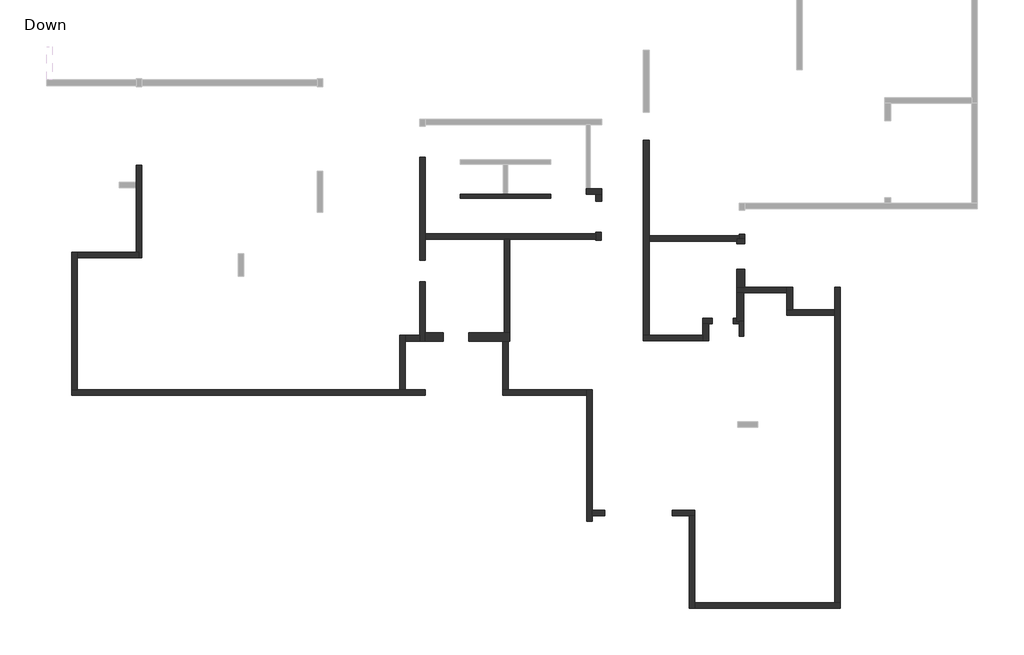
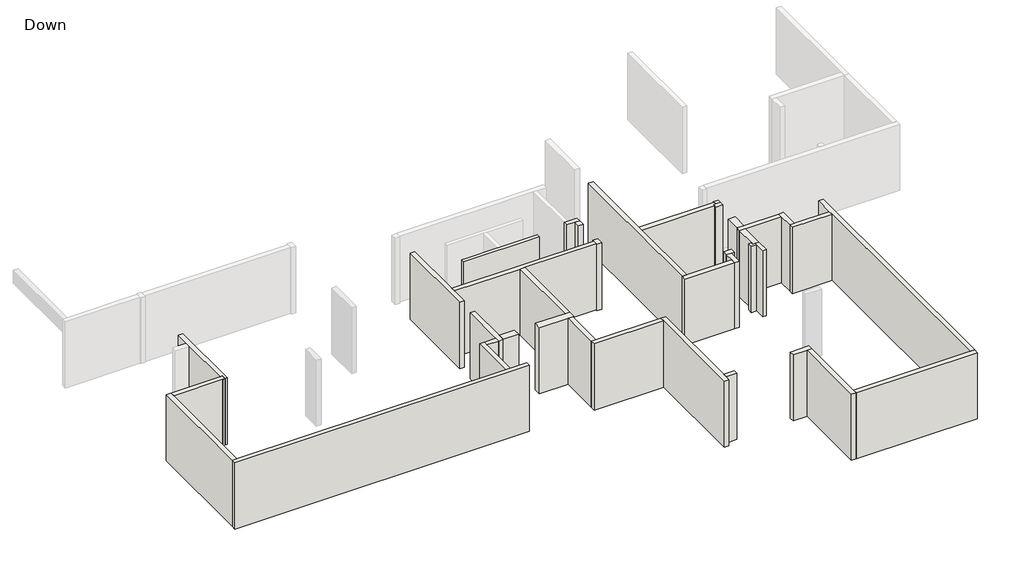
# One storey, part 1 of 3: 38 walls.
"""IFC4 building model written with IfcOpenShell, lengths in millimetres."""

from ifc_helpers import new_model, si_unit, origin, place, context, project, spatial, faceted_brep, element, save

model = new_model("IFC4")

# Units and contexts
model_context = context("Model", 3, world=origin())
ifc_project = project(units=[si_unit("LENGTHUNIT", "METRE", prefix="MILLI")], contexts=[model_context])

# Site, building, storey
site = spatial("IfcSite", under=ifc_project)
building = spatial("IfcBuilding", under=site)
storey = spatial("IfcBuildingStorey", under=building, Name="Down", Elevation=0.0)

# Walls
placement = place(None, origin())
element("IfcWall", 1, ObjectType="15", at=placement, inside=storey, context=model_context, shape_type="Brep", body=[
    faceted_brep([(8929.8987326, -5377.2065162, 0.0), (8929.8987326, -4829.2179242, 0.0), (8929.8987326, -4829.2179242, 3000.0), (8929.8987326, -5377.2065162, 3000.0), (8929.8987326, -5377.2065162, 2800.0), (8779.8987326, -5377.2065162, 0.0), (8779.8987326, -5377.2065162, 2800.0), (8779.8987326, -5377.2065162, 3000.0), (8779.8987326, -4929.2179242, 3000.0), (8779.8987326, -4829.2179242, 3000.0), (8779.8987326, -4829.2179242, 0.0), (8779.8987326, -4929.2179242, 0.0)], [[[0, 1, 2, 3, 4]], [[5, 6, 7, 8, 9, 10, 11]], [[1, 0, 5, 11, 10]], [[2, 1, 10, 9]], [[3, 2, 9, 8, 7]], [[0, 4, 3, 7, 6, 5]]]),
])
element("IfcWall", 2, ObjectType="15", at=placement, inside=storey, context=model_context, shape_type="Brep", body=[
    faceted_brep([(2055.2627374, -306.6458737, 0.0), (511.0080091, -306.6458737, 0.0), (361.0080091, -306.6458737, 0.0), (-1185.5058006, -306.6458737, 0.0), (-1185.5058006, -306.6458737, 2800.0), (-1185.5058006, -306.6458737, 3000.0), (-985.5058006, -306.6458737, 3000.0), (361.0080091, -306.6458737, 3000.0), (511.0080091, -306.6458737, 3000.0), (1795.2627374, -306.6458737, 3000.0), (2055.2627374, -306.6458737, 3000.0), (2055.2627374, -306.6458737, 2800.0), (2055.2627374, -456.6458737, 0.0), (2055.2627374, -456.6458737, 2800.0), (2055.2627374, -456.6458737, 3000.0), (-1185.5058006, -456.6458737, 3000.0), (-1185.5058006, -456.6458737, 2800.0), (-1185.5058006, -456.6458737, 0.0)], [[[0, 1, 2, 3, 4, 5, 6, 7, 8, 9, 10, 11]], [[12, 13, 14, 15, 16, 17]], [[3, 2, 1, 0, 12, 17]], [[5, 4, 3, 17, 16, 15]], [[10, 9, 8, 7, 6, 5, 15, 14]], [[0, 11, 10, 14, 13, 12]]]),
])
element("IfcWall", 3, ObjectType="20", at=placement, inside=storey, context=model_context, shape_type="Brep", body=[
    faceted_brep([(3525.3580541, -11777.7243787, 0.0), (3983.0434339, -11777.7243787, 0.0), (3983.0434339, -11777.7243787, 2800.0), (3983.0434339, -11777.7243787, 3000.0), (3525.3580541, -11777.7243787, 3000.0), (3525.3580541, -11777.7243787, 2800.0), (3525.3580541, -11577.7243787, 0.0), (3525.3580541, -11577.7243787, 2800.0), (3525.3580541, -11577.7243787, 3000.0), (3983.0434339, -11577.7243787, 3000.0), (3983.0434339, -11577.7243787, 2800.0), (3983.0434339, -11577.7243787, 0.0)], [[[0, 1, 2, 3, 4, 5]], [[6, 7, 8, 9, 10, 11]], [[1, 0, 6, 11]], [[3, 2, 1, 11, 10, 9]], [[4, 3, 9, 8]], [[0, 5, 4, 8, 7, 6]]]),
])
element("IfcWall", 4, ObjectType="20", at=placement, inside=storey, context=model_context, shape_type="Brep", body=[
    faceted_brep([(6385.0248209, -11777.7243787, 0.0), (6985.0248209, -11777.7243787, 0.0), (7185.0248209, -11777.7243787, 0.0), (7185.0248209, -11777.7243787, 3000.0), (6985.0248209, -11777.7243787, 3000.0), (6385.0248209, -11777.7243787, 3000.0), (6385.0248209, -11777.7243787, 2800.0), (6385.0248209, -11577.7243787, 0.0), (6385.0248209, -11577.7243787, 2800.0), (6385.0248209, -11577.7243787, 3000.0), (7185.0248209, -11577.7243787, 3000.0), (7185.0248209, -11577.7243787, 2800.0), (7185.0248209, -11577.7243787, 0.0)], [[[0, 1, 2, 3, 4, 5, 6]], [[7, 8, 9, 10, 11, 12]], [[2, 1, 0, 7, 12]], [[5, 4, 3, 10, 9]], [[0, 6, 5, 9, 8, 7]], [[3, 2, 12, 11, 10]]]),
])
element("IfcWall", 5, ObjectType="20", at=placement, inside=storey, context=model_context, shape_type="Brep", body=[
    faceted_brep([(6985.0248209, -11777.7243787, 0.0), (6985.0248209, -15077.7243787, 0.0), (6985.0248209, -15077.7243787, 3000.0), (6985.0248209, -14877.7243787, 3000.0), (6985.0248209, -11777.7243787, 3000.0), (6985.0248209, -11777.7243787, 2800.0), (7185.0248209, -11777.7243787, 0.0), (7185.0248209, -11777.7243787, 3000.0), (7185.0248209, -14877.7243787, 3000.0), (7185.0248209, -15077.7243787, 3000.0), (7185.0248209, -15077.7243787, 0.0), (7185.0248209, -14877.7243787, 0.0)], [[[0, 1, 2, 3, 4, 5]], [[6, 7, 8, 9, 10, 11]], [[1, 0, 6, 11, 10]], [[4, 3, 2, 9, 8, 7]], [[0, 5, 4, 7, 6]], [[2, 1, 10, 9]]]),
])
element("IfcWall", 6, ObjectType="20", at=placement, inside=storey, context=model_context, shape_type="Brep", body=[
    faceted_brep([(7185.0248209, -15077.7243787, 0.0), (12385.0248209, -15077.7243787, 0.0), (12385.0248209, -15077.7243787, 3000.0), (7185.0248209, -15077.7243787, 3000.0), (7185.0248209, -14877.7243787, 0.0), (7185.0248209, -14877.7243787, 2800.0), (7185.0248209, -14877.7243787, 3000.0), (12185.0248209, -14877.7243787, 3000.0), (12385.0248209, -14877.7243787, 3000.0), (12385.0248209, -14877.7243787, 0.0), (12185.0248209, -14877.7243787, 0.0)], [[[0, 1, 2, 3]], [[4, 5, 6, 7, 8, 9, 10]], [[1, 0, 4, 10, 9]], [[3, 2, 8, 7, 6]], [[0, 3, 6, 5, 4]], [[2, 1, 9, 8]]]),
])
element("IfcWall", 7, ObjectType="20", at=placement, inside=storey, context=model_context, shape_type="Brep", body=[
    faceted_brep([(12385.0248209, -14877.7243787, 0.0), (12385.0248209, -3627.7243787, 0.0), (12385.0248209, -3627.7243787, 3000.0), (12385.0248209, -14877.7243787, 3000.0), (12185.0248209, -14877.7243787, 0.0), (12185.0248209, -14877.7243787, 2800.0), (12185.0248209, -14877.7243787, 3000.0), (12185.0248209, -4626.5873327, 3000.0), (12185.0248209, -4426.5873327, 3000.0), (12185.0248209, -3627.7243787, 3000.0), (12185.0248209, -3627.7243787, 0.0), (12185.0248209, -4426.5873327, 0.0), (12185.0248209, -4626.5873327, 0.0)], [[[0, 1, 2, 3]], [[4, 5, 6, 7, 8, 9, 10, 11, 12]], [[1, 0, 4, 12, 11, 10]], [[2, 1, 10, 9]], [[3, 2, 9, 8, 7, 6]], [[0, 3, 6, 5, 4]]]),
])
element("IfcWall", 8, ObjectType="20", at=placement, inside=storey, context=model_context, shape_type="Brep", body=[
    faceted_brep([(10478.8780181, -4626.5873327, 0.0), (12185.0248209, -4626.5873327, 0.0), (12185.0248209, -4626.5873327, 2800.0), (12185.0248209, -4626.5873327, 3000.0), (10478.8780181, -4626.5873327, 3000.0), (10478.8780181, -4626.5873327, 2800.0), (10478.8780181, -4426.5873327, 0.0), (10478.8780181, -4426.5873327, 3000.0), (10678.8780181, -4426.5873327, 3000.0), (12185.0248209, -4426.5873327, 3000.0), (12185.0248209, -4426.5873327, 0.0), (10678.8780181, -4426.5873327, 0.0)], [[[0, 1, 2, 3, 4, 5]], [[6, 7, 8, 9, 10, 11]], [[1, 0, 6, 11, 10]], [[4, 3, 9, 8, 7]], [[3, 2, 1, 10, 9]], [[0, 5, 4, 7, 6]]]),
])
element("IfcWall", 9, ObjectType="20", at=placement, inside=storey, context=model_context, shape_type="Brep", body=[
    faceted_brep([(10678.8780181, -4426.5873327, 0.0), (10678.8780181, -3625.7617548, 0.0), (10678.8780181, -3625.7617548, 3000.0), (10678.8780181, -4426.5873327, 3000.0), (10478.8780181, -4426.5873327, 0.0), (10478.8780181, -4426.5873327, 3000.0), (10478.8780181, -3825.7617548, 3000.0), (10478.8780181, -3625.7617548, 3000.0), (10478.8780181, -3625.7617548, 0.0), (10478.8780181, -3825.7617548, 0.0)], [[[0, 1, 2, 3]], [[4, 5, 6, 7, 8, 9]], [[1, 0, 4, 9, 8]], [[3, 2, 7, 6, 5]], [[2, 1, 8, 7]], [[0, 3, 5, 4]]]),
])
element("IfcWall", 10, ObjectType="20", at=placement, inside=storey, context=model_context, shape_type="Brep", body=[
    faceted_brep([(10478.8780181, -3625.7617548, 0.0), (8979.7748959, -3625.7617548, 0.0), (8679.9812904, -3625.7617548, 0.0), (8679.9812904, -3625.7617548, 2800.0), (8679.9812904, -3625.7617548, 3000.0), (8979.7748959, -3625.7617548, 3000.0), (10478.8780181, -3625.7617548, 3000.0), (10478.8780181, -3825.7617548, 0.0), (10478.8780181, -3825.7617548, 2800.0), (10478.8780181, -3825.7617548, 3000.0), (8929.9812904, -3825.7617548, 3000.0), (8679.9812904, -3825.7617548, 3000.0), (8679.9812904, -3825.7617548, 0.0), (8929.9812904, -3825.7617548, 0.0)], [[[0, 1, 2, 3, 4, 5, 6]], [[7, 8, 9, 10, 11, 12, 13]], [[2, 1, 0, 7, 13, 12]], [[6, 5, 4, 11, 10, 9]], [[0, 6, 9, 8, 7]], [[4, 3, 2, 12, 11]]]),
])
element("IfcWall", 11, ObjectType="20", at=placement, inside=storey, context=model_context, shape_type="Brep", body=[
    faceted_brep([(8679.9812904, -4729.2179242, 0.0), (8554.8987326, -4729.2179242, 0.0), (8554.8987326, -4729.2179242, 2800.0), (8554.8987326, -4729.2179242, 3000.0), (8679.9812904, -4729.2179242, 3000.0), (8779.8987326, -4929.2179242, 0.0), (8779.8987326, -4929.2179242, 2800.0), (8779.8987326, -4929.2179242, 3000.0), (8554.8987326, -4929.2179242, 3000.0), (8554.8987326, -4929.2179242, 2800.0), (8554.8987326, -4929.2179242, 0.0), (8679.9812904, -4829.2179242, 0.0), (8779.8987326, -4829.2179242, 0.0), (8779.8987326, -4829.2179242, 3000.0), (8679.9812904, -4829.2179242, 3000.0)], [[[0, 1, 2, 3, 4]], [[5, 6, 7, 8, 9, 10]], [[1, 0, 11, 12, 5, 10]], [[3, 2, 1, 10, 9, 8]], [[4, 3, 8, 7, 13, 14]], [[0, 4, 14, 11]], [[14, 13, 12, 11]], [[13, 7, 6, 5, 12]]]),
])
element("IfcWall", 12, ObjectType="20", at=placement, inside=storey, context=model_context, shape_type="Brep", body=[
    faceted_brep([(7481.1671205, -4929.2179242, 0.0), (7481.1671205, -5329.7132709, 0.0), (7481.1671205, -5529.7132709, 0.0), (7481.1671205, -5529.7132709, 3000.0), (7481.1671205, -5329.7132709, 3000.0), (7481.1671205, -4929.2179242, 3000.0), (7681.1671205, -4929.2179242, 0.0), (7681.1671205, -4929.2179242, 2800.0), (7681.1671205, -4929.2179242, 3000.0), (7681.1671205, -5529.7132709, 3000.0), (7681.1671205, -5529.7132709, 2800.0), (7681.1671205, -5529.7132709, 0.0)], [[[0, 1, 2, 3, 4, 5]], [[6, 7, 8, 9, 10, 11]], [[2, 1, 0, 6, 11]], [[5, 4, 3, 9, 8]], [[3, 2, 11, 10, 9]], [[0, 5, 8, 7, 6]]]),
])
element("IfcWall", 13, ObjectType="20", at=placement, inside=storey, context=model_context, shape_type="Brep", body=[
    faceted_brep([(7481.1671205, -5329.7132709, 0.0), (5555.6042265, -5329.7132709, 0.0), (5355.6042265, -5329.7132709, 0.0), (5355.6042265, -5329.7132709, 3000.0), (5555.6042265, -5329.7132709, 3000.0), (7481.1671205, -5329.7132709, 3000.0), (7481.1671205, -5329.7132709, 2800.0), (7481.1671205, -5529.7132709, 0.0), (7481.1671205, -5529.7132709, 3000.0), (5355.6042265, -5529.7132709, 3000.0), (5355.6042265, -5529.7132709, 2800.0), (5355.6042265, -5529.7132709, 0.0)], [[[0, 1, 2, 3, 4, 5, 6]], [[7, 8, 9, 10, 11]], [[2, 1, 0, 7, 11]], [[5, 4, 3, 9, 8]], [[0, 6, 5, 8, 7]], [[3, 2, 11, 10, 9]]]),
])
element("IfcWall", 14, ObjectType="20", at=placement, inside=storey, context=model_context, shape_type="Brep", body=[
    faceted_brep([(5555.6042265, -5329.7132709, 0.0), (5555.6042265, -1979.0002718, 0.0), (5555.6042265, -1779.0002718, 0.0), (5555.6042265, 1623.6415775, 0.0), (5555.6042265, 1623.6415775, 2800.0), (5555.6042265, 1623.6415775, 3000.0), (5555.6042265, -1779.0002718, 3000.0), (5555.6042265, -1979.0002718, 3000.0), (5555.6042265, -5329.7132709, 3000.0), (5555.6042265, -5329.7132709, 2800.0), (5355.6042265, -5329.7132709, 0.0), (5355.6042265, -5329.7132709, 3000.0), (5355.6042265, -1955.5013225, 3000.0), (5355.6042265, -560.9043547, 3000.0), (5355.6042265, 1623.6415775, 3000.0), (5355.6042265, 1623.6415775, 2800.0), (5355.6042265, 1623.6415775, 0.0)], [[[0, 1, 2, 3, 4, 5, 6, 7, 8, 9]], [[10, 11, 12, 13, 14, 15, 16]], [[3, 2, 1, 0, 10, 16]], [[5, 4, 3, 16, 15, 14]], [[8, 7, 6, 5, 14, 13, 12, 11]], [[0, 9, 8, 11, 10]]]),
])
element("IfcWall", 15, ObjectType="20", at=placement, inside=storey, context=model_context, shape_type="Brep", body=[
    faceted_brep([(5555.6042265, -1979.0002718, 0.0), (8679.7748959, -1979.0002718, 0.0), (8679.7748959, -1979.0002718, 2800.0), (8679.7748959, -1979.0002718, 3000.0), (5555.6042265, -1979.0002718, 3000.0), (5555.6042265, -1979.0002718, 2800.0), (5555.6042265, -1779.0002718, 0.0), (5555.6042265, -1779.0002718, 2800.0), (5555.6042265, -1779.0002718, 3000.0), (8779.7748959, -1779.0002718, 3000.0), (8779.7748959, -1779.0002718, 2800.0), (8779.7748959, -1779.0002718, 0.0), (8779.7748959, -1879.0002718, 0.0), (8679.7748959, -1879.0002718, 0.0), (8679.7748959, -1879.0002718, 3000.0), (8779.7748959, -1879.0002718, 3000.0)], [[[0, 1, 2, 3, 4, 5]], [[6, 7, 8, 9, 10, 11]], [[1, 0, 6, 11, 12, 13]], [[4, 3, 14, 15, 9, 8]], [[3, 2, 1, 13, 14]], [[13, 12, 15, 14]], [[12, 11, 10, 9, 15]], [[0, 5, 4, 8, 7, 6]]]),
])
element("IfcWall", 16, ObjectType="20", at=placement, inside=storey, context=model_context, shape_type="Brep", body=[
    faceted_brep([(3525.3580541, -11977.8894943, 0.0), (3525.3580541, -11777.7243787, 0.0), (3525.3580541, -11577.7243787, 0.0), (3525.3580541, -7276.5573117, 0.0), (3525.3580541, -7276.5573117, 2800.0), (3525.3580541, -7276.5573117, 3000.0), (3525.3580541, -11577.7243787, 3000.0), (3525.3580541, -11777.7243787, 3000.0), (3525.3580541, -11977.8894943, 3000.0), (3525.3580541, -11977.8894943, 2400.0), (3325.3580541, -11977.8894943, 0.0), (3325.3580541, -11977.8894943, 2400.0), (3325.3580541, -11977.8894943, 3000.0), (3325.3580541, -7476.5573117, 3000.0), (3325.3580541, -7276.5573117, 3000.0), (3325.3580541, -7276.5573117, 0.0), (3325.3580541, -7476.5573117, 0.0)], [[[0, 1, 2, 3, 4, 5, 6, 7, 8, 9]], [[10, 11, 12, 13, 14, 15, 16]], [[3, 2, 1, 0, 10, 16, 15]], [[8, 7, 6, 5, 14, 13, 12]], [[0, 9, 8, 12, 11, 10]], [[5, 4, 3, 15, 14]]]),
])
element("IfcWall", 17, ObjectType="20", at=placement, inside=storey, context=model_context, shape_type="Brep", body=[
    faceted_brep([(3325.3580541, -7276.5573117, 0.0), (539.5617467, -7276.5573117, 0.0), (339.5617467, -7276.5573117, 0.0), (339.5617467, -7276.5573117, 3000.0), (539.5617467, -7276.5573117, 3000.0), (3325.3580541, -7276.5573117, 3000.0), (3325.3580541, -7476.5573117, 0.0), (3325.3580541, -7476.5573117, 3000.0), (339.5617467, -7476.5573117, 3000.0), (339.5617467, -7476.5573117, 0.0)], [[[0, 1, 2, 3, 4, 5]], [[6, 7, 8, 9]], [[2, 1, 0, 6, 9]], [[5, 4, 3, 8, 7]], [[3, 2, 9, 8]], [[0, 5, 7, 6]]]),
])
element("IfcWall", 18, ObjectType="20", at=placement, inside=storey, context=model_context, shape_type="Brep", body=[
    faceted_brep([(539.5617467, -7276.5573117, 0.0), (539.5617467, -5546.2285816, 0.0), (539.5617467, -5546.2285816, 2800.0), (539.5617467, -5546.2285816, 3000.0), (539.5617467, -7276.5573117, 3000.0), (539.5617467, -7276.5573117, 2800.0), (339.5617467, -7276.5573117, 0.0), (339.5617467, -7276.5573117, 3000.0), (339.5617467, -5546.2285816, 3000.0), (339.5617467, -5546.2285816, 0.0)], [[[0, 1, 2, 3, 4, 5]], [[6, 7, 8, 9]], [[1, 0, 6, 9]], [[4, 3, 8, 7]], [[0, 5, 4, 7, 6]], [[3, 2, 1, 9, 8]]]),
])
element("IfcWall", 19, ObjectType="20", at=placement, inside=storey, context=model_context, shape_type="Brep", body=[
    faceted_brep([(-2431.7719369, -7276.5573117, 0.0), (-3134.897875, -7276.5573117, 0.0), (-3334.897875, -7276.5573117, 0.0), (-14851.7058906, -7276.5573117, 0.0), (-15051.7058906, -7276.5573117, 0.0), (-15051.7058906, -7276.5573117, 3000.0), (-14851.7058906, -7276.5573117, 3000.0), (-3334.897875, -7276.5573117, 3000.0), (-3134.897875, -7276.5573117, 3000.0), (-2431.7719369, -7276.5573117, 3000.0), (-2431.7719369, -7476.5573117, 0.0), (-2431.7719369, -7476.5573117, 3000.0), (-15051.7058906, -7476.5573117, 3000.0), (-15051.7058906, -7476.5573117, 0.0)], [[[0, 1, 2, 3, 4, 5, 6, 7, 8, 9]], [[10, 11, 12, 13]], [[4, 3, 2, 1, 0, 10, 13]], [[9, 8, 7, 6, 5, 12, 11]], [[0, 9, 11, 10]], [[5, 4, 13, 12]]]),
])
element("IfcWall", 20, ObjectType="20", at=placement, inside=storey, context=model_context, shape_type="Brep", body=[
    faceted_brep([(-14851.7058906, -7276.5573117, 0.0), (-14851.7058906, -2576.5573117, 0.0), (-14851.7058906, -2376.5573117, 0.0), (-14851.7058906, -2376.5573117, 3000.0), (-14851.7058906, -2576.5573117, 3000.0), (-14851.7058906, -7276.5573117, 3000.0), (-14851.7058906, -7276.5573117, 2800.0), (-15051.7058906, -7276.5573117, 0.0), (-15051.7058906, -7276.5573117, 3000.0), (-15051.7058906, -2376.5573117, 3000.0), (-15051.7058906, -2376.5573117, 0.0)], [[[0, 1, 2, 3, 4, 5, 6]], [[7, 8, 9, 10]], [[2, 1, 0, 7, 10]], [[5, 4, 3, 9, 8]], [[0, 6, 5, 8, 7]], [[3, 2, 10, 9]]]),
])
element("IfcWall", 21, ObjectType="20", at=placement, inside=storey, context=model_context, shape_type="Brep", body=[
    faceted_brep([(-14851.7058906, -2576.5573117, 0.0), (-12744.8761098, -2576.5573117, 0.0), (-12645.0412254, -2576.5573117, 0.0), (-12645.0412254, -2576.5573117, 3000.0), (-12744.8761098, -2576.5573117, 3000.0), (-14851.7058906, -2576.5573117, 3000.0), (-14851.7058906, -2576.5573117, 2800.0), (-14851.7058906, -2376.5573117, 0.0), (-14851.7058906, -2376.5573117, 3000.0), (-12744.8761098, -2376.5573117, 3000.0), (-12645.0412254, -2376.5573117, 3000.0), (-12645.0412254, -2376.5573117, 0.0), (-12744.8761098, -2376.5573117, 0.0)], [[[0, 1, 2, 3, 4, 5, 6]], [[7, 8, 9, 10, 11, 12]], [[2, 1, 0, 7, 12, 11]], [[3, 2, 11, 10]], [[5, 4, 3, 10, 9, 8]], [[0, 6, 5, 8, 7]]]),
])
element("IfcWall", 22, ObjectType="20", at=placement, inside=storey, context=model_context, shape_type="Brep", body=[
    faceted_brep([(-12544.8761098, -2576.936327, 0.0), (-12544.8761098, 723.063673, 0.0), (-12544.8761098, 723.063673, 2800.0), (-12544.8761098, 723.063673, 3000.0), (-12544.8761098, -2576.936327, 3000.0), (-12544.8761098, -2576.936327, 2800.0), (-12744.8761098, 723.063673, 3000.0), (-12744.8761098, 723.063673, 2800.0), (-12744.8761098, 723.063673, 0.0), (-12744.8761098, 117.6373746, 0.0), (-12744.8761098, -82.3626254, 0.0), (-12744.8761098, -2376.5573117, 0.0), (-12744.8761098, -2376.5573117, 3000.0), (-12744.8761098, -82.3626254, 3000.0), (-12744.8761098, 117.6373746, 3000.0), (-12744.8761098, -2576.936327, 0.0), (-12744.8761098, -2576.936327, 2800.0), (-12744.8761098, -2576.936327, 3000.0), (-12744.8761098, -2576.5573117, 3000.0), (-12744.8761098, -2576.5573117, 2800.0), (-12744.8761098, -2576.5573117, 0.0), (-12645.0412254, -2576.5573117, 0.0), (-12645.0412254, -2376.5573117, 0.0), (-12645.0412254, -2376.5573117, 3000.0), (-12645.0412254, -2576.5573117, 3000.0)], [[[0, 1, 2, 3, 4, 5]], [[6, 7, 8, 9, 10, 11, 12, 13, 14]], [[15, 16, 17, 18, 19, 20]], [[1, 0, 15, 20, 21, 22, 11, 10, 9, 8]], [[3, 2, 1, 8, 7, 6]], [[4, 3, 6, 14, 13, 12, 23, 24, 18, 17]], [[0, 5, 4, 17, 16, 15]], [[24, 21, 20, 19, 18]], [[22, 23, 12, 11]], [[21, 24, 23, 22]]]),
])
element("IfcWall", 23, ObjectType="20", at=placement, inside=storey, context=model_context, shape_type="Brep", body=[
    faceted_brep([(-3334.897875, -5346.2285816, 0.0), (-3334.897875, -7276.5573117, 0.0), (-3334.897875, -7276.5573117, 2800.0), (-3334.897875, -7276.5573117, 3000.0), (-3334.897875, -5346.2285816, 3000.0), (-3334.897875, -5346.2285816, 2800.0), (-3134.897875, -5346.2285816, 0.0), (-3134.897875, -5346.2285816, 3000.0), (-3134.897875, -5546.2285816, 3000.0), (-3134.897875, -7276.5573117, 3000.0), (-3134.897875, -7276.5573117, 0.0), (-3134.897875, -5546.2285816, 0.0)], [[[0, 1, 2, 3, 4, 5]], [[6, 7, 8, 9, 10, 11]], [[1, 0, 6, 11, 10]], [[4, 3, 9, 8, 7]], [[0, 5, 4, 7, 6]], [[3, 2, 1, 10, 9]]]),
])
element("IfcWall", 24, ObjectType="20", at=placement, inside=storey, context=model_context, shape_type="Brep", body=[
    faceted_brep([(-3134.897875, -5546.2285816, 0.0), (-2634.3199705, -5546.2285816, 0.0), (-2634.3199705, -5546.2285816, 3000.0), (-3134.897875, -5546.2285816, 3000.0), (-3134.897875, -5346.2285816, 0.0), (-3134.897875, -5346.2285816, 3000.0), (-2634.3199705, -5346.2285816, 3000.0), (-2634.3199705, -5346.2285816, 2800.0), (-2634.3199705, -5346.2285816, 0.0)], [[[0, 1, 2, 3]], [[4, 5, 6, 7, 8]], [[1, 0, 4, 8]], [[3, 2, 6, 5]], [[0, 3, 5, 4]], [[2, 1, 8, 7, 6]]]),
])
element("IfcWall", 25, ObjectType="20", at=placement, inside=storey, context=model_context, shape_type="Brep", body=[
    faceted_brep([(-2634.3199705, -3430.3624753, 0.0), (-2634.3199705, -5346.2285816, 0.0), (-2634.3199705, -5546.2285816, 0.0), (-2634.3199705, -5546.2285816, 3000.0), (-2634.3199705, -5346.2285816, 3000.0), (-2634.3199705, -3430.3624753, 3000.0), (-2634.3199705, -3430.3624753, 2800.0), (-2434.3199705, -3430.3624753, 0.0), (-2434.3199705, -3430.3624753, 2800.0), (-2434.3199705, -3430.3624753, 3000.0), (-2434.3199705, -5246.2285816, 3000.0), (-2434.3199705, -5546.2285816, 3000.0), (-2434.3199705, -5546.2285816, 0.0), (-2434.3199705, -5246.2285816, 0.0)], [[[0, 1, 2, 3, 4, 5, 6]], [[7, 8, 9, 10, 11, 12, 13]], [[2, 1, 0, 7, 13, 12]], [[5, 4, 3, 11, 10, 9]], [[0, 6, 5, 9, 8, 7]], [[3, 2, 12, 11]]]),
])
element("IfcWall", 26, ObjectType="20", at=placement, inside=storey, context=model_context, shape_type="Brep", body=[
    faceted_brep([(585.0023051, -5246.2285816, 0.0), (585.0023051, -1909.5654174, 0.0), (585.0023051, -1909.5654174, 2800.0), (585.0023051, -1909.5654174, 3000.0), (585.0023051, -5246.2285816, 3000.0), (385.0023051, -5246.2285816, 0.0), (385.0023051, -5246.2285816, 2800.0), (385.0023051, -5246.2285816, 3000.0), (385.0023051, -1909.5654174, 3000.0), (385.0023051, -1909.5654174, 2800.0), (385.0023051, -1909.5654174, 0.0)], [[[0, 1, 2, 3, 4]], [[5, 6, 7, 8, 9, 10]], [[1, 0, 5, 10]], [[4, 3, 8, 7]], [[0, 4, 7, 6, 5]], [[3, 2, 1, 10, 9, 8]]]),
])
element("IfcWall", 27, ObjectType="20", at=placement, inside=storey, context=model_context, shape_type="Brep", body=[
    faceted_brep([(3654.3658596, -1709.5654174, 0.0), (-2434.3199705, -1709.5654174, 0.0), (-2434.3199705, -1709.5654174, 2800.0), (-2434.3199705, -1709.5654174, 3000.0), (3654.3658596, -1709.5654174, 3000.0), (3654.3658596, -1709.5654174, 2800.0), (3654.3658596, -1909.5654174, 0.0), (3654.3658596, -1909.5654174, 2800.0), (3654.3658596, -1909.5654174, 3000.0), (585.0023051, -1909.5654174, 3000.0), (385.0023051, -1909.5654174, 3000.0), (-2434.3199705, -1909.5654174, 3000.0), (-2434.3199705, -1909.5654174, 2800.0), (-2434.3199705, -1909.5654174, 0.0), (385.0023051, -1909.5654174, 0.0), (585.0023051, -1909.5654174, 0.0)], [[[0, 1, 2, 3, 4, 5]], [[6, 7, 8, 9, 10, 11, 12, 13, 14, 15]], [[1, 0, 6, 15, 14, 13]], [[4, 3, 11, 10, 9, 8]], [[0, 5, 4, 8, 7, 6]], [[3, 2, 1, 13, 12, 11]]]),
])
element("IfcWall", 28, ObjectType="20", at=placement, inside=storey, context=model_context, shape_type="Brep", body=[
    faceted_brep([(8779.7748959, -1726.7411904, 0.0), (8779.7748959, -1779.0002718, 0.0), (8779.7748959, -1879.0002718, 0.0), (8779.7748959, -1879.0002718, 3000.0), (8779.7748959, -1779.0002718, 3000.0), (8779.7748959, -1726.7411904, 3000.0), (8779.7748959, -1726.7411904, 2800.0), (8979.7748959, -1726.7411904, 0.0), (8979.7748959, -1726.7411904, 3000.0), (8979.7748959, -1879.0002718, 3000.0), (8979.7748959, -1879.0002718, 0.0)], [[[0, 1, 2, 3, 4, 5, 6]], [[7, 8, 9, 10]], [[2, 1, 0, 7, 10]], [[3, 2, 10, 9]], [[5, 4, 3, 9, 8]], [[0, 6, 5, 8, 7]]]),
])
element("IfcWall", 29, ObjectType="20", at=placement, inside=storey, context=model_context, shape_type="Brep", body=[
    faceted_brep([(7481.1671205, -4929.2179242, 0.0), (7681.1671205, -4929.2179242, 0.0), (7809.9023103, -4929.2179242, 0.0), (7809.9023103, -4929.2179242, 2800.0), (7809.9023103, -4929.2179242, 3000.0), (7681.1671205, -4929.2179242, 3000.0), (7481.1671205, -4929.2179242, 3000.0), (7481.1671205, -4729.2179242, 0.0), (7481.1671205, -4729.2179242, 2800.0), (7481.1671205, -4729.2179242, 3000.0), (7809.9023103, -4729.2179242, 3000.0), (7809.9023103, -4729.2179242, 2800.0), (7809.9023103, -4729.2179242, 0.0)], [[[0, 1, 2, 3, 4, 5, 6]], [[7, 8, 9, 10, 11, 12]], [[2, 1, 0, 7, 12]], [[4, 3, 2, 12, 11, 10]], [[6, 5, 4, 10, 9]], [[0, 6, 9, 8, 7]]]),
])
element("IfcWall", 30, ObjectType="20", at=placement, inside=storey, context=model_context, shape_type="Brep", body=[
    faceted_brep([(-2434.3199705, -2660.6799476, 0.0), (-2434.3199705, -1909.5654174, 0.0), (-2434.3199705, -1709.5654174, 0.0), (-2434.3199705, 1012.4872695, 0.0), (-2434.3199705, 1012.4872695, 2800.0), (-2434.3199705, 1012.4872695, 3000.0), (-2434.3199705, -1709.5654174, 3000.0), (-2434.3199705, -1909.5654174, 3000.0), (-2434.3199705, -2660.6799476, 3000.0), (-2434.3199705, -2660.6799476, 2800.0), (-2634.3199705, -2660.6799476, 0.0), (-2634.3199705, -2660.6799476, 2800.0), (-2634.3199705, -2660.6799476, 3000.0), (-2634.3199705, 1012.4872695, 3000.0), (-2634.3199705, 1012.4872695, 2800.0), (-2634.3199705, 1012.4872695, 0.0)], [[[0, 1, 2, 3, 4, 5, 6, 7, 8, 9]], [[10, 11, 12, 13, 14, 15]], [[3, 2, 1, 0, 10, 15]], [[5, 4, 3, 15, 14, 13]], [[8, 7, 6, 5, 13, 12]], [[0, 9, 8, 12, 11, 10]]]),
])
element("IfcWall", 31, ObjectType="20", at=placement, inside=storey, context=model_context, shape_type="Brep", body=[
    faceted_brep([(3311.0605459, -305.9043547, 0.0), (3661.0605459, -305.9043547, 0.0), (3861.0605459, -305.9043547, 0.0), (3861.0605459, -305.9043547, 3000.0), (3661.0605459, -305.9043547, 3000.0), (3311.0605459, -305.9043547, 3000.0), (3311.0605459, -305.9043547, 2800.0), (3311.0605459, -105.9043547, 0.0), (3311.0605459, -105.9043547, 3000.0), (3461.0605459, -105.9043547, 3000.0), (3861.0605459, -105.9043547, 3000.0), (3861.0605459, -105.9043547, 2800.0), (3861.0605459, -105.9043547, 0.0), (3461.0605459, -105.9043547, 0.0)], [[[0, 1, 2, 3, 4, 5, 6]], [[7, 8, 9, 10, 11, 12, 13]], [[2, 1, 0, 7, 13, 12]], [[5, 4, 3, 10, 9, 8]], [[0, 6, 5, 8, 7]], [[3, 2, 12, 11, 10]]]),
])
element("IfcWall", 32, ObjectType="20", at=placement, inside=storey, context=model_context, shape_type="Brep", body=[
    faceted_brep([(3661.0605459, -305.9043547, 0.0), (3661.0605459, -560.9043547, 0.0), (3661.0605459, -560.9043547, 2800.0), (3661.0605459, -560.9043547, 3000.0), (3661.0605459, -305.9043547, 3000.0), (3661.0605459, -305.9043547, 2800.0), (3861.0605459, -305.9043547, 0.0), (3861.0605459, -305.9043547, 3000.0), (3861.0605459, -560.9043547, 3000.0), (3861.0605459, -560.9043547, 2800.0), (3861.0605459, -560.9043547, 0.0)], [[[0, 1, 2, 3, 4, 5]], [[6, 7, 8, 9, 10]], [[1, 0, 6, 10]], [[3, 2, 1, 10, 9, 8]], [[4, 3, 8, 7]], [[0, 5, 4, 7, 6]]]),
])
element("IfcWall", 33, ObjectType="20", at=placement, inside=storey, context=model_context, shape_type="Brep", body=[
    faceted_brep([(3654.3658596, -1655.2536492, 0.0), (3654.3658596, -1709.5654174, 0.0), (3654.3658596, -1909.5654174, 0.0), (3654.3658596, -1955.5013225, 0.0), (3654.3658596, -1955.5013225, 2800.0), (3654.3658596, -1955.5013225, 3000.0), (3654.3658596, -1909.5654174, 3000.0), (3654.3658596, -1709.5654174, 3000.0), (3654.3658596, -1655.2536492, 3000.0), (3654.3658596, -1655.2536492, 2800.0), (3854.3658596, -1655.2536492, 0.0), (3854.3658596, -1655.2536492, 2800.0), (3854.3658596, -1655.2536492, 3000.0), (3854.3658596, -1955.5013225, 3000.0), (3854.3658596, -1955.5013225, 2800.0), (3854.3658596, -1955.5013225, 0.0)], [[[0, 1, 2, 3, 4, 5, 6, 7, 8, 9]], [[10, 11, 12, 13, 14, 15]], [[3, 2, 1, 0, 10, 15]], [[5, 4, 3, 15, 14, 13]], [[8, 7, 6, 5, 13, 12]], [[0, 9, 8, 12, 11, 10]]]),
])
element("IfcWall", 34, ObjectType="25", at=placement, inside=storey, context=model_context, shape_type="Brep", body=[
    faceted_brep([(8679.9812904, -3825.7617548, 0.0), (8679.9812904, -4729.2179242, 0.0), (8679.9812904, -4829.2179242, 0.0), (8679.9812904, -4829.2179242, 3000.0), (8679.9812904, -4729.2179242, 3000.0), (8679.9812904, -3825.7617548, 3000.0), (8929.9812904, -3825.7617548, 0.0), (8929.9812904, -3825.7617548, 2800.0), (8929.9812904, -3825.7617548, 3000.0), (8929.9812904, -4829.2179242, 3000.0), (8929.9812904, -4829.2179242, 0.0), (8779.8987326, -4829.2179242, 0.0), (8779.8987326, -4829.2179242, 3000.0)], [[[0, 1, 2, 3, 4, 5]], [[6, 7, 8, 9, 10]], [[2, 1, 0, 6, 10, 11]], [[3, 2, 11, 10, 9, 12]], [[5, 4, 3, 12, 9, 8]], [[0, 5, 8, 7, 6]]]),
])
element("IfcWall", 35, ObjectType="30", at=placement, inside=storey, context=model_context, shape_type="Brep", body=[
    faceted_brep([(8679.7748959, -2977.6080472, 0.0), (8679.7748959, -3625.7617548, 0.0), (8679.7748959, -3625.7617548, 2800.0), (8679.7748959, -3625.7617548, 3000.0), (8679.7748959, -2977.6080472, 3000.0), (8679.7748959, -2977.6080472, 2800.0), (8979.7748959, -2977.6080472, 0.0), (8979.7748959, -2977.6080472, 2800.0), (8979.7748959, -2977.6080472, 3000.0), (8979.7748959, -3625.7617548, 3000.0), (8979.7748959, -3625.7617548, 0.0), (8679.9812904, -3625.7617548, 0.0), (8679.9812904, -3625.7617548, 3000.0)], [[[0, 1, 2, 3, 4, 5]], [[6, 7, 8, 9, 10]], [[1, 0, 6, 10, 11]], [[4, 3, 12, 9, 8]], [[0, 5, 4, 8, 7, 6]], [[3, 2, 1, 11, 10, 9, 12]]]),
])
element("IfcWall", 36, ObjectType="30", at=placement, inside=storey, context=model_context, shape_type="Brep", body=[
    faceted_brep([(-2434.3199705, -5546.2285816, 0.0), (-1781.9370524, -5546.2285816, 0.0), (-1781.9370524, -5546.2285816, 2800.0), (-1781.9370524, -5546.2285816, 3000.0), (-2434.3199705, -5546.2285816, 3000.0), (-2434.3199705, -5246.2285816, 0.0), (-2434.3199705, -5246.2285816, 2800.0), (-2434.3199705, -5246.2285816, 3000.0), (-1781.9370524, -5246.2285816, 3000.0), (-1781.9370524, -5246.2285816, 2800.0), (-1781.9370524, -5246.2285816, 0.0)], [[[0, 1, 2, 3, 4]], [[5, 6, 7, 8, 9, 10]], [[1, 0, 5, 10]], [[3, 2, 1, 10, 9, 8]], [[4, 3, 8, 7]], [[0, 4, 7, 6, 5]]]),
])
element("IfcWall", 37, ObjectType="30", at=placement, inside=storey, context=model_context, shape_type="Brep", body=[
    faceted_brep([(-885.2581272, -5546.2285816, 0.0), (339.5617467, -5546.2285816, 0.0), (539.5617467, -5546.2285816, 0.0), (585.0023051, -5546.2285816, 0.0), (585.0023051, -5546.2285816, 2800.0), (585.0023051, -5546.2285816, 3000.0), (539.5617467, -5546.2285816, 3000.0), (339.5617467, -5546.2285816, 3000.0), (-885.2581272, -5546.2285816, 3000.0), (-885.2581272, -5546.2285816, 2800.0), (-885.2581272, -5246.2285816, 0.0), (-885.2581272, -5246.2285816, 2800.0), (-885.2581272, -5246.2285816, 3000.0), (385.0023051, -5246.2285816, 3000.0), (585.0023051, -5246.2285816, 3000.0), (585.0023051, -5246.2285816, 0.0), (385.0023051, -5246.2285816, 0.0)], [[[0, 1, 2, 3, 4, 5, 6, 7, 8, 9]], [[10, 11, 12, 13, 14, 15, 16]], [[3, 2, 1, 0, 10, 16, 15]], [[8, 7, 6, 5, 14, 13, 12]], [[0, 9, 8, 12, 11, 10]], [[5, 4, 3, 15, 14]]]),
])
element("IfcWall", 38, ObjectType="30", at=placement, inside=storey, context=model_context, shape_type="Brep", body=[
    faceted_brep([(8679.7748959, -1879.0002718, 0.0), (8679.7748959, -1979.0002718, 0.0), (8679.7748959, -2077.0301427, 0.0), (8679.7748959, -2077.0301427, 2800.0), (8679.7748959, -2077.0301427, 3000.0), (8679.7748959, -1979.0002718, 3000.0), (8679.7748959, -1879.0002718, 3000.0), (8979.7748959, -1879.0002718, 0.0), (8979.7748959, -1879.0002718, 3000.0), (8979.7748959, -2077.0301427, 3000.0), (8979.7748959, -2077.0301427, 2800.0), (8979.7748959, -2077.0301427, 0.0), (8779.7748959, -1879.0002718, 0.0), (8779.7748959, -1879.0002718, 3000.0)], [[[0, 1, 2, 3, 4, 5, 6]], [[7, 8, 9, 10, 11]], [[2, 1, 0, 12, 7, 11]], [[4, 3, 2, 11, 10, 9]], [[6, 5, 4, 9, 8, 13]], [[0, 6, 13, 8, 7, 12]]]),
])

save(model, "model.ifc")

# Revit data of these elements
# Project information
#   Project Issue Date = "Issue Date"
#   Project Status = "Project Status"
#   Client Name = "לקוח"
#   Project Address = "Enter address here"
#   Project Name = "Project 015"
#   Project Number = "מספר פרויקט"
# Type "15"
#   Layers, outside or top first: 15 cm "Concrete" (function 1)
# Type "20"
#   Layers, outside or top first: 20 cm "Concrete" (function 1)
# Type "25"
#   Layers, outside or top first: 25 cm "Concrete" (function 1)
# Type "30"
#   Layers, outside or top first: 30 cm "Concrete" (function 1)
# Element 1 (IfcWall, "15")
#   Comments = ""
#   Mark = "W100"
#   SOFiSTiK_EdgeZones = "W100"
#   SOFiSTiK_AMG_Comments = ""
#   Top Offset = 0 cm
#   Base Offset = 0 cm
#   wall height = 300 cm
#   SOFiSTiK_AMG_Scheduled = yes
#   SOFiSTiK_AMG_Adjusted = yes
#   Phase Created = New Construction
#   Base Constraint = Down
#   Top Constraint = Typical Floor
#   Materials on its faces: "Concrete"
# Element 2 (IfcWall, "15")
#   Comments = ""
#   Mark = "W107"
#   SOFiSTiK_EdgeZones = "W107"
#   SOFiSTiK_AMG_Comments = ""
#   Top Offset = 0 cm
#   Base Offset = 0 cm
#   wall height = 300 cm
#   SOFiSTiK_AMG_Scheduled = yes
#   SOFiSTiK_AMG_Adjusted = yes
#   Phase Created = New Construction
#   Base Constraint = Down
#   Top Constraint = Typical Floor
#   Materials on its faces: "Concrete"
# Element 3 (IfcWall, "20")
#   Comments = ""
#   Mark = "W45"
#   SOFiSTiK_EdgeZones = "W45"
#   SOFiSTiK_AMG_Comments = ""
#   Top Offset = 0 cm
#   Base Offset = 0 cm
#   wall height = 300 cm
#   SOFiSTiK_AMG_Scheduled = yes
#   SOFiSTiK_AMG_Adjusted = yes
#   Phase Created = New Construction
#   Base Constraint = Down
#   Top Constraint = Typical Floor
#   Materials on its faces: "Concrete"
# Element 4 (IfcWall, "20")
#   Comments = ""
#   Mark = "W46"
#   SOFiSTiK_EdgeZones = "W46"
#   SOFiSTiK_AMG_Comments = ""
#   Top Offset = 0 cm
#   Base Offset = 0 cm
#   wall height = 300 cm
#   SOFiSTiK_AMG_Scheduled = yes
#   SOFiSTiK_AMG_Adjusted = yes
#   Phase Created = New Construction
#   Base Constraint = Down
#   Top Constraint = Typical Floor
#   Materials on its faces: "Concrete"
# Element 5 (IfcWall, "20")
#   Comments = ""
#   Mark = "W47"
#   SOFiSTiK_EdgeZones = "W47"
#   SOFiSTiK_AMG_Comments = ""
#   Top Offset = 0 cm
#   Base Offset = 0 cm
#   wall height = 300 cm
#   SOFiSTiK_AMG_Scheduled = yes
#   SOFiSTiK_AMG_Adjusted = yes
#   Phase Created = New Construction
#   Base Constraint = Down
#   Top Constraint = Typical Floor
#   Materials on its faces: "Concrete"
# Element 6 (IfcWall, "20")
#   Comments = ""
#   Mark = "W48"
#   SOFiSTiK_EdgeZones = "W48"
#   SOFiSTiK_AMG_Comments = ""
#   Top Offset = 0 cm
#   Base Offset = 0 cm
#   wall height = 300 cm
#   SOFiSTiK_AMG_Scheduled = yes
#   SOFiSTiK_AMG_Adjusted = yes
#   Phase Created = New Construction
#   Base Constraint = Down
#   Top Constraint = Typical Floor
#   Materials on its faces: "Concrete"
# Element 7 (IfcWall, "20")
#   Comments = ""
#   Mark = "W49"
#   SOFiSTiK_EdgeZones = "W49"
#   SOFiSTiK_AMG_Comments = ""
#   Top Offset = 0 cm
#   Base Offset = 0 cm
#   wall height = 300 cm
#   SOFiSTiK_AMG_Scheduled = yes
#   SOFiSTiK_AMG_Adjusted = yes
#   Phase Created = New Construction
#   Base Constraint = Down
#   Top Constraint = Typical Floor
#   Materials on its faces: "Concrete"
# Element 8 (IfcWall, "20")
#   Comments = ""
#   Mark = "W50"
#   SOFiSTiK_EdgeZones = "W50"
#   SOFiSTiK_AMG_Comments = ""
#   Top Offset = 0 cm
#   Base Offset = 0 cm
#   wall height = 300 cm
#   SOFiSTiK_AMG_Scheduled = yes
#   SOFiSTiK_AMG_Adjusted = yes
#   Phase Created = New Construction
#   Base Constraint = Down
#   Top Constraint = Typical Floor
#   Materials on its faces: "Concrete"
# Element 9 (IfcWall, "20")
#   Comments = ""
#   Mark = "W51"
#   SOFiSTiK_EdgeZones = "W51"
#   SOFiSTiK_AMG_Comments = ""
#   Top Offset = 0 cm
#   Base Offset = 0 cm
#   wall height = 300 cm
#   SOFiSTiK_AMG_Scheduled = yes
#   SOFiSTiK_AMG_Adjusted = yes
#   Phase Created = New Construction
#   Base Constraint = Down
#   Top Constraint = Typical Floor
#   Materials on its faces: "Concrete"
# Element 10 (IfcWall, "20")
#   Comments = ""
#   Mark = "W52"
#   SOFiSTiK_EdgeZones = "W52"
#   SOFiSTiK_AMG_Comments = ""
#   Top Offset = 0 cm
#   Base Offset = 0 cm
#   wall height = 300 cm
#   SOFiSTiK_AMG_Scheduled = yes
#   SOFiSTiK_AMG_Adjusted = yes
#   Phase Created = New Construction
#   Base Constraint = Down
#   Top Constraint = Typical Floor
#   Materials on its faces: "Concrete"
# Element 11 (IfcWall, "20")
#   Comments = ""
#   Mark = "W53"
#   SOFiSTiK_EdgeZones = "W53"
#   SOFiSTiK_AMG_Comments = ""
#   Top Offset = 0 cm
#   Base Offset = 0 cm
#   wall height = 300 cm
#   SOFiSTiK_AMG_Scheduled = yes
#   SOFiSTiK_AMG_Adjusted = yes
#   Phase Created = New Construction
#   Base Constraint = Down
#   Top Constraint = Typical Floor
#   Materials on its faces: "Concrete"
# Element 12 (IfcWall, "20")
#   Comments = ""
#   Mark = "W54"
#   SOFiSTiK_EdgeZones = "W54"
#   SOFiSTiK_AMG_Comments = ""
#   Top Offset = 0 cm
#   Base Offset = 0 cm
#   wall height = 300 cm
#   SOFiSTiK_AMG_Scheduled = yes
#   SOFiSTiK_AMG_Adjusted = yes
#   Phase Created = New Construction
#   Base Constraint = Down
#   Top Constraint = Typical Floor
#   Materials on its faces: "Concrete"
# Element 13 (IfcWall, "20")
#   Comments = ""
#   Mark = "W55"
#   SOFiSTiK_EdgeZones = "W55"
#   SOFiSTiK_AMG_Comments = ""
#   Top Offset = 0 cm
#   Base Offset = 0 cm
#   wall height = 300 cm
#   SOFiSTiK_AMG_Scheduled = yes
#   SOFiSTiK_AMG_Adjusted = yes
#   Phase Created = New Construction
#   Base Constraint = Down
#   Top Constraint = Typical Floor
#   Materials on its faces: "Concrete"
# Element 14 (IfcWall, "20")
#   Comments = ""
#   Mark = "W56"
#   SOFiSTiK_EdgeZones = "W56"
#   SOFiSTiK_AMG_Comments = ""
#   Top Offset = 0 cm
#   Base Offset = 0 cm
#   wall height = 300 cm
#   SOFiSTiK_AMG_Scheduled = yes
#   SOFiSTiK_AMG_Adjusted = yes
#   Phase Created = New Construction
#   Base Constraint = Down
#   Top Constraint = Typical Floor
#   Materials on its faces: "Concrete"
# Element 15 (IfcWall, "20")
#   Comments = ""
#   Mark = "W57"
#   SOFiSTiK_EdgeZones = "W57"
#   SOFiSTiK_AMG_Comments = ""
#   Top Offset = 0 cm
#   Base Offset = 0 cm
#   wall height = 300 cm
#   SOFiSTiK_AMG_Scheduled = yes
#   SOFiSTiK_AMG_Adjusted = yes
#   Phase Created = New Construction
#   Base Constraint = Down
#   Top Constraint = Typical Floor
#   Materials on its faces: "Concrete"
# Element 16 (IfcWall, "20")
#   Comments = ""
#   Mark = "W61"
#   SOFiSTiK_EdgeZones = "W61"
#   SOFiSTiK_AMG_Comments = ""
#   Top Offset = 0 cm
#   Base Offset = 0 cm
#   wall height = 300 cm
#   SOFiSTiK_AMG_Scheduled = yes
#   SOFiSTiK_AMG_Adjusted = yes
#   Phase Created = New Construction
#   Base Constraint = Down
#   Top Constraint = Typical Floor
#   Materials on its faces: "Concrete"
# Element 17 (IfcWall, "20")
#   Comments = ""
#   Mark = "W63"
#   SOFiSTiK_EdgeZones = "W63"
#   SOFiSTiK_AMG_Comments = ""
#   Top Offset = 0 cm
#   Base Offset = 0 cm
#   wall height = 300 cm
#   SOFiSTiK_AMG_Scheduled = yes
#   SOFiSTiK_AMG_Adjusted = yes
#   Phase Created = New Construction
#   Base Constraint = Down
#   Top Constraint = Typical Floor
#   Materials on its faces: "Concrete"
# Element 18 (IfcWall, "20")
#   Comments = ""
#   Mark = "W64"
#   SOFiSTiK_EdgeZones = "W64"
#   SOFiSTiK_AMG_Comments = ""
#   Top Offset = 0 cm
#   Base Offset = 0 cm
#   wall height = 300 cm
#   SOFiSTiK_AMG_Scheduled = yes
#   SOFiSTiK_AMG_Adjusted = yes
#   Phase Created = New Construction
#   Base Constraint = Down
#   Top Constraint = Typical Floor
#   Materials on its faces: "Concrete"
# Element 19 (IfcWall, "20")
#   Comments = ""
#   Mark = "W65"
#   SOFiSTiK_EdgeZones = "W65"
#   SOFiSTiK_AMG_Comments = ""
#   Top Offset = 0 cm
#   Base Offset = 0 cm
#   wall height = 300 cm
#   SOFiSTiK_AMG_Scheduled = yes
#   SOFiSTiK_AMG_Adjusted = yes
#   Phase Created = New Construction
#   Base Constraint = Down
#   Top Constraint = Typical Floor
#   Materials on its faces: "Concrete"
# Element 20 (IfcWall, "20")
#   Comments = ""
#   Mark = "W66"
#   SOFiSTiK_EdgeZones = "W66"
#   SOFiSTiK_AMG_Comments = ""
#   Top Offset = 0 cm
#   Base Offset = 0 cm
#   wall height = 300 cm
#   SOFiSTiK_AMG_Scheduled = yes
#   SOFiSTiK_AMG_Adjusted = yes
#   Phase Created = New Construction
#   Base Constraint = Down
#   Top Constraint = Typical Floor
#   Materials on its faces: "Concrete"
# Element 21 (IfcWall, "20")
#   Comments = ""
#   Mark = "W67"
#   SOFiSTiK_EdgeZones = "W67"
#   SOFiSTiK_AMG_Comments = ""
#   Top Offset = 0 cm
#   Base Offset = 0 cm
#   wall height = 300 cm
#   SOFiSTiK_AMG_Scheduled = yes
#   SOFiSTiK_AMG_Adjusted = yes
#   Phase Created = New Construction
#   Base Constraint = Down
#   Top Constraint = Typical Floor
#   Materials on its faces: "Concrete"
# Element 22 (IfcWall, "20")
#   Comments = ""
#   Mark = "W69"
#   SOFiSTiK_EdgeZones = "W69"
#   SOFiSTiK_AMG_Comments = ""
#   Top Offset = 0 cm
#   Base Offset = 0 cm
#   wall height = 300 cm
#   SOFiSTiK_AMG_Scheduled = yes
#   SOFiSTiK_AMG_Adjusted = yes
#   Phase Created = New Construction
#   Base Constraint = Down
#   Top Constraint = Typical Floor
#   Materials on its faces: "Concrete"
# Element 23 (IfcWall, "20")
#   Comments = ""
#   Mark = "W71"
#   SOFiSTiK_EdgeZones = "W71"
#   SOFiSTiK_AMG_Comments = ""
#   Top Offset = 0 cm
#   Base Offset = 0 cm
#   wall height = 300 cm
#   SOFiSTiK_AMG_Scheduled = yes
#   SOFiSTiK_AMG_Adjusted = yes
#   Phase Created = New Construction
#   Base Constraint = Down
#   Top Constraint = Typical Floor
#   Materials on its faces: "Concrete"
# Element 24 (IfcWall, "20")
#   Comments = ""
#   Mark = "W72"
#   SOFiSTiK_EdgeZones = "W72"
#   SOFiSTiK_AMG_Comments = ""
#   Top Offset = 0 cm
#   Base Offset = 0 cm
#   wall height = 300 cm
#   SOFiSTiK_AMG_Scheduled = yes
#   SOFiSTiK_AMG_Adjusted = yes
#   Phase Created = New Construction
#   Base Constraint = Down
#   Top Constraint = Typical Floor
#   Materials on its faces: "Concrete"
# Element 25 (IfcWall, "20")
#   Comments = ""
#   Mark = "W73"
#   SOFiSTiK_EdgeZones = "W73"
#   SOFiSTiK_AMG_Comments = ""
#   Top Offset = 0 cm
#   Base Offset = 0 cm
#   wall height = 300 cm
#   SOFiSTiK_AMG_Scheduled = yes
#   SOFiSTiK_AMG_Adjusted = yes
#   Phase Created = New Construction
#   Base Constraint = Down
#   Top Constraint = Typical Floor
#   Materials on its faces: "Concrete"
# Element 26 (IfcWall, "20")
#   Comments = ""
#   Mark = "W74"
#   SOFiSTiK_EdgeZones = "W74"
#   SOFiSTiK_AMG_Comments = ""
#   Top Offset = 0 cm
#   Base Offset = 0 cm
#   wall height = 300 cm
#   SOFiSTiK_AMG_Scheduled = yes
#   SOFiSTiK_AMG_Adjusted = yes
#   Phase Created = New Construction
#   Base Constraint = Down
#   Top Constraint = Typical Floor
#   Materials on its faces: "Concrete"
# Element 27 (IfcWall, "20")
#   Comments = ""
#   Mark = "W75"
#   SOFiSTiK_EdgeZones = "W75"
#   SOFiSTiK_AMG_Comments = ""
#   Top Offset = 0 cm
#   Base Offset = 0 cm
#   wall height = 300 cm
#   SOFiSTiK_AMG_Scheduled = yes
#   SOFiSTiK_AMG_Adjusted = yes
#   Phase Created = New Construction
#   Base Constraint = Down
#   Top Constraint = Typical Floor
#   Materials on its faces: "Concrete"
# Element 28 (IfcWall, "20")
#   Comments = ""
#   Mark = "W80"
#   SOFiSTiK_EdgeZones = "W80"
#   SOFiSTiK_AMG_Comments = ""
#   Top Offset = 0 cm
#   Base Offset = 0 cm
#   wall height = 300 cm
#   SOFiSTiK_AMG_Scheduled = yes
#   SOFiSTiK_AMG_Adjusted = yes
#   Phase Created = New Construction
#   Base Constraint = Down
#   Top Constraint = Typical Floor
#   Materials on its faces: "Concrete"
# Element 29 (IfcWall, "20")
#   Comments = ""
#   Mark = "W81"
#   SOFiSTiK_EdgeZones = "W81"
#   SOFiSTiK_AMG_Comments = ""
#   Top Offset = 0 cm
#   Base Offset = 0 cm
#   wall height = 300 cm
#   SOFiSTiK_AMG_Scheduled = yes
#   SOFiSTiK_AMG_Adjusted = yes
#   Phase Created = New Construction
#   Base Constraint = Down
#   Top Constraint = Typical Floor
#   Materials on its faces: "Concrete"
# Element 30 (IfcWall, "20")
#   Comments = ""
#   Mark = "W88"
#   SOFiSTiK_EdgeZones = "W88"
#   SOFiSTiK_AMG_Comments = ""
#   Top Offset = 0 cm
#   Base Offset = 0 cm
#   wall height = 300 cm
#   SOFiSTiK_AMG_Scheduled = yes
#   SOFiSTiK_AMG_Adjusted = yes
#   Phase Created = New Construction
#   Base Constraint = Down
#   Top Constraint = Typical Floor
#   Materials on its faces: "Concrete"
# Element 31 (IfcWall, "20")
#   Comments = ""
#   Mark = "W91"
#   SOFiSTiK_EdgeZones = "W91"
#   SOFiSTiK_AMG_Comments = ""
#   Top Offset = 0 cm
#   Base Offset = 0 cm
#   wall height = 300 cm
#   SOFiSTiK_AMG_Scheduled = yes
#   SOFiSTiK_AMG_Adjusted = yes
#   Phase Created = New Construction
#   Base Constraint = Down
#   Top Constraint = Typical Floor
#   Materials on its faces: "Concrete"
# Element 32 (IfcWall, "20")
#   Comments = ""
#   Mark = "W92"
#   SOFiSTiK_EdgeZones = "W92"
#   SOFiSTiK_AMG_Comments = ""
#   Top Offset = 0 cm
#   Base Offset = 0 cm
#   wall height = 300 cm
#   SOFiSTiK_AMG_Scheduled = yes
#   SOFiSTiK_AMG_Adjusted = yes
#   Phase Created = New Construction
#   Base Constraint = Down
#   Top Constraint = Typical Floor
#   Materials on its faces: "Concrete"
# Element 33 (IfcWall, "20")
#   Comments = ""
#   Mark = "W93"
#   SOFiSTiK_EdgeZones = "W93"
#   SOFiSTiK_AMG_Comments = ""
#   Top Offset = 0 cm
#   Base Offset = 0 cm
#   wall height = 300 cm
#   SOFiSTiK_AMG_Scheduled = yes
#   SOFiSTiK_AMG_Adjusted = yes
#   Phase Created = New Construction
#   Base Constraint = Down
#   Top Constraint = Typical Floor
#   Materials on its faces: "Concrete"
# Element 34 (IfcWall, "25")
#   Comments = ""
#   Mark = "W98"
#   SOFiSTiK_EdgeZones = "W98"
#   SOFiSTiK_AMG_Comments = ""
#   Top Offset = 0 cm
#   Base Offset = 0 cm
#   wall height = 300 cm
#   SOFiSTiK_AMG_Scheduled = yes
#   SOFiSTiK_AMG_Adjusted = yes
#   Phase Created = New Construction
#   Base Constraint = Down
#   Top Constraint = Typical Floor
#   Materials on its faces: "Concrete"
# Element 35 (IfcWall, "30")
#   Comments = ""
#   Mark = "W111"
#   SOFiSTiK_EdgeZones = "W111"
#   SOFiSTiK_AMG_Comments = ""
#   Top Offset = 0 cm
#   Base Offset = 0 cm
#   wall height = 300 cm
#   SOFiSTiK_AMG_Scheduled = yes
#   SOFiSTiK_AMG_Adjusted = yes
#   Phase Created = New Construction
#   Base Constraint = Down
#   Top Constraint = Typical Floor
#   Materials on its faces: "Concrete"
# Element 36 (IfcWall, "30")
#   Comments = ""
#   Mark = "W112"
#   SOFiSTiK_EdgeZones = "W112"
#   SOFiSTiK_AMG_Comments = ""
#   Top Offset = 0 cm
#   Base Offset = 0 cm
#   wall height = 300 cm
#   SOFiSTiK_AMG_Scheduled = yes
#   SOFiSTiK_AMG_Adjusted = yes
#   Phase Created = New Construction
#   Base Constraint = Down
#   Top Constraint = Typical Floor
#   Materials on its faces: "Concrete"
# Element 37 (IfcWall, "30")
#   Comments = ""
#   Mark = "W113"
#   SOFiSTiK_EdgeZones = "W113"
#   SOFiSTiK_AMG_Comments = ""
#   Top Offset = 0 cm
#   Base Offset = 0 cm
#   wall height = 300 cm
#   SOFiSTiK_AMG_Scheduled = yes
#   SOFiSTiK_AMG_Adjusted = yes
#   Phase Created = New Construction
#   Base Constraint = Down
#   Top Constraint = Typical Floor
#   Materials on its faces: "Concrete"
# Element 38 (IfcWall, "30")
#   Comments = ""
#   Mark = "W114"
#   SOFiSTiK_EdgeZones = "W114"
#   SOFiSTiK_AMG_Comments = ""
#   Top Offset = 0 cm
#   Base Offset = 0 cm
#   wall height = 300 cm
#   SOFiSTiK_AMG_Scheduled = yes
#   SOFiSTiK_AMG_Adjusted = yes
#   Phase Created = New Construction
#   Base Constraint = Down
#   Top Constraint = Typical Floor
#   Materials on its faces: "Concrete"
# Materials
#   "Concrete": class "Concrete", colour RGB 192 192 192, transparency 0, Keynote = "01000", Description = "Cast-in-place concrete", Cost = 0
